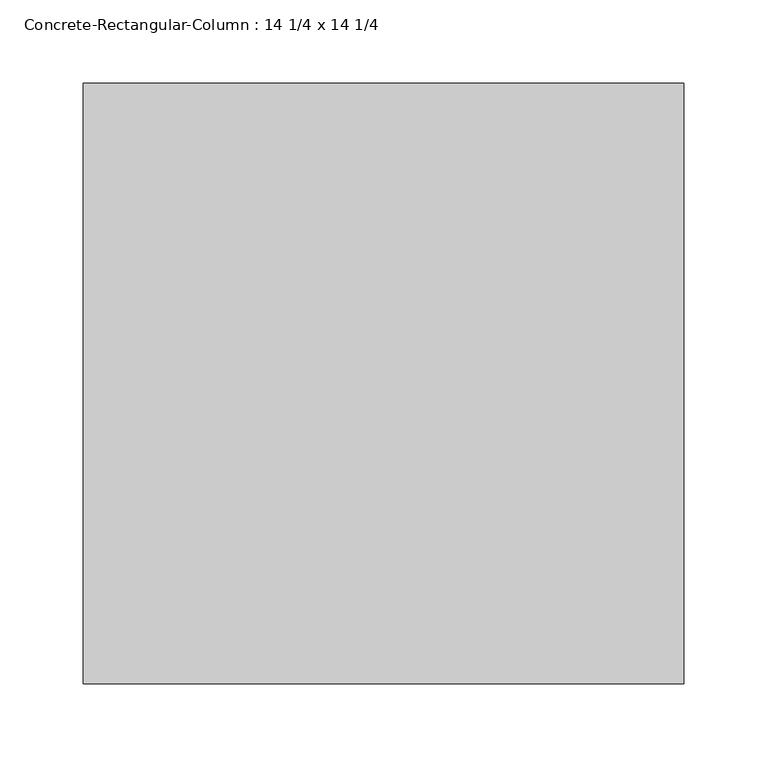
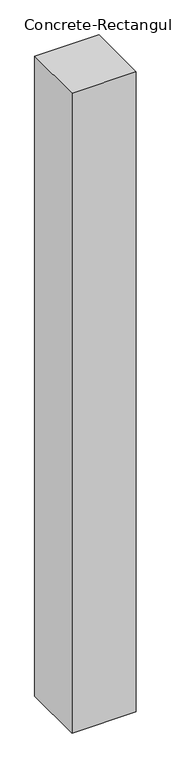
"""IFC4 building model written with IfcOpenShell, lengths in millimetres: column geometry, Concrete-Rectangular-Column : 14 1/4 x 14 1/4."""

import ifcopenshell
import ifcopenshell.guid

model = None  # the IFC model being written
_history = None  # IfcOwnerHistory: only IFC2X3 demands one
_inside = {}  # id of a spatial element -> (the spatial element, [elements in it])
_under = {}  # id of a project, library or spatial element -> (it, [spatial elements below it])
_declared = {}  # id of a project -> (the project, [libraries it declares])
_typed = {}  # id of a type object -> (the type object, [elements of that type])
_made_of = {}  # id of a material, layer set ... -> (it, [elements and type objects made of it])


def new_model(schema):
    """Start an empty IFC model of exactly this schema.

    Asked for "IFC4X3", IfcOpenShell would pick the latest addendum, in which some entities
    have other attributes; the version numbers below select the first issue.
    IFC2X3 requires an IfcOwnerHistory on every rooted entity: one is made here for all.
    """
    global model, _history
    if schema == "IFC4X3":
        model = ifcopenshell.file(schema_version=(4, 3, 0, 0))
    else:
        model = ifcopenshell.file(schema=schema)
    _inside.clear()
    _under.clear()
    _declared.clear()
    _typed.clear()
    _made_of.clear()
    _history = None
    if model.schema == "IFC2X3":
        org = make("IfcOrganization", Name="unknown")
        user = make(
            "IfcPersonAndOrganization",
            ThePerson=make("IfcPerson", FamilyName="unknown"),
            TheOrganization=org,
        )
        app = make(
            "IfcApplication",
            ApplicationDeveloper=org,
            Version="unknown",
            ApplicationFullName="unknown",
            ApplicationIdentifier="unknown",
        )
        _history = make(
            "IfcOwnerHistory",
            OwningUser=user,
            OwningApplication=app,
            ChangeAction="ADDED",
            CreationDate=0,
        )
    return model


def make(cls, **values):
    """One entity of the class cls with the attributes given. An attribute that is None is left unset."""
    return model.create_entity(
        cls, **{name: value for name, value in values.items() if value is not None}
    )


def rooted(cls, **values):
    """An entity with a GlobalId (a new one), such as an element, a storey or a relation."""
    return make(cls, GlobalId=ifcopenshell.guid.new(), OwnerHistory=_history, **values)


def si_unit(unit_type, name, prefix=None):
    """IfcSIUnit, for example si_unit("LENGTHUNIT", "METRE", prefix="MILLI")."""
    return make("IfcSIUnit", UnitType=unit_type, Prefix=prefix, Name=name)


def assignment(units):
    """IfcUnitAssignment: the units of a project."""
    return None if units is None else make("IfcUnitAssignment", Units=units)


def point(xyz):
    """IfcCartesianPoint."""
    return None if xyz is None else make("IfcCartesianPoint", Coordinates=xyz)


def direction(xyz):
    """IfcDirection."""
    return None if xyz is None else make("IfcDirection", DirectionRatios=xyz)


def frame(location, z_axis=None, x_axis=None):
    """IfcAxis2Placement3D, a coordinate frame: its origin and axes. An axis left out is left unset."""
    return make(
        "IfcAxis2Placement3D",
        Location=point(location),
        Axis=direction(z_axis),
        RefDirection=direction(x_axis),
    )


def origin():
    """The frame at (0, 0, 0) with its axes left unset."""
    return frame((0.0, 0.0, 0.0))


def origin_with_axes():
    """The frame at (0, 0, 0) with the z axis (0, 0, 1) and the x axis (1, 0, 0) written out."""
    return frame((0.0, 0.0, 0.0), z_axis=(0.0, 0.0, 1.0), x_axis=(1.0, 0.0, 0.0))


def place(relative_to, where):
    """IfcLocalPlacement: puts the frame where relative to a parent placement (None: the world)."""
    return make(
        "IfcLocalPlacement", PlacementRelTo=relative_to, RelativePlacement=where
    )


def context(
    kind, dimensions, precision=None, world=None, true_north=None, identifier=None
):
    """IfcGeometricRepresentationContext, for example the 3D "Model" context."""
    return make(
        "IfcGeometricRepresentationContext",
        ContextIdentifier=identifier,
        ContextType=kind,
        CoordinateSpaceDimension=dimensions,
        Precision=precision,
        WorldCoordinateSystem=world,
        TrueNorth=true_north,
    )


def project(units=None, contexts=None):
    """IfcProject with its units and contexts."""
    return rooted(
        "IfcProject",
        Name="project",
        RepresentationContexts=contexts,
        UnitsInContext=assignment(units),
    )


def spatial(cls, under=None, at=None, **own):
    """A site, building, storey or space (cls), placed at a placement, below another one or the project."""
    s = rooted(cls, ObjectPlacement=at, **own)
    if under is not None:
        _under.setdefault(under.id(), (under, []))[1].append(s)
    return s


def polyline(points):
    """IfcPolyline through the points."""
    return make("IfcPolyline", Points=[point(p) for p in points])


def outline(outer, holes=None, kind="AREA"):
    """IfcArbitraryClosedProfileDef: a profile drawn as a closed curve; with holes, ...WithVoids."""
    if holes is None:
        return make("IfcArbitraryClosedProfileDef", ProfileType=kind, OuterCurve=outer)
    return make(
        "IfcArbitraryProfileDefWithVoids",
        ProfileType=kind,
        OuterCurve=outer,
        InnerCurves=holes,
    )


def extrude(swept, where, along, depth):
    """IfcExtrudedAreaSolid: the profile swept, set in the frame where, extruded along a direction by depth."""
    return make(
        "IfcExtrudedAreaSolid",
        SweptArea=swept,
        Position=where,
        ExtrudedDirection=direction(along),
        Depth=depth,
    )


def shape(context_of_items, identifier, shape_type, items):
    """IfcShapeRepresentation: the items that make up one representation, for example the "Body"."""
    return make(
        "IfcShapeRepresentation",
        ContextOfItems=context_of_items,
        RepresentationIdentifier=identifier,
        RepresentationType=shape_type,
        Items=items,
    )


def source(mapping_origin, context_of_items, identifier, shape_type, items):
    """IfcRepresentationMap: a shape defined once, which mapped items show again and again."""
    return make(
        "IfcRepresentationMap",
        MappingOrigin=mapping_origin,
        MappedRepresentation=shape(context_of_items, identifier, shape_type, items),
    )


def transform(
    local_origin,
    x_axis=None,
    y_axis=None,
    z_axis=None,
    scale=None,
    scale2=None,
    scale3=None,
    uniform=True,
):
    """IfcCartesianTransformationOperator3D, or its non-uniform kind. x_axis, y_axis, z_axis: its Axis1, 2, 3."""
    if uniform:
        return make(
            "IfcCartesianTransformationOperator3D",
            Axis1=direction(x_axis),
            Axis2=direction(y_axis),
            LocalOrigin=point(local_origin),
            Scale=scale,
            Axis3=direction(z_axis),
        )
    return make(
        "IfcCartesianTransformationOperator3DnonUniform",
        Axis1=direction(x_axis),
        Axis2=direction(y_axis),
        LocalOrigin=point(local_origin),
        Scale=scale,
        Axis3=direction(z_axis),
        Scale2=scale2,
        Scale3=scale3,
    )


def mapped(mapping_source, mapping_target):
    """IfcMappedItem: shows the shape of a source again, moved by a transform."""
    return make(
        "IfcMappedItem", MappingSource=mapping_source, MappingTarget=mapping_target
    )


def made_of(thing, what):
    """Note that an element or type object is made of a material, layer set ...; save() writes the relation."""
    if what is not None:
        _made_of.setdefault(what.id(), (what, []))[1].append(thing)
    return thing


def element(
    cls,
    number,
    at=None,
    inside=None,
    cuts=None,
    type_object=None,
    material=None,
    context=None,
    identifier="Body",
    shape_type=None,
    held_by="IfcProductDefinitionShape",
    body=None,
    shapes=None,
    **own,
):
    """One element of the class cls, such as IfcWall. Its Tag is "e" and its number.

    at: its placement. inside: the storey or other place that contains it. cuts: it is an
    opening in that element (IfcRelVoidsElement). A single representation is given by context,
    identifier, shape_type and body (its items); several are given by shapes. held_by: the class
    of the entity that holds the representations. save() writes the other relations.
    """
    e = rooted(cls, Tag="e%d" % number, ObjectPlacement=at, **own)
    if body is not None:
        shapes = [shape(context, identifier, shape_type, body)]
    if shapes is not None:
        e.Representation = make(held_by, Representations=shapes)
    if inside is not None:
        _inside.setdefault(inside.id(), (inside, []))[1].append(e)
    if cuts is not None:
        rooted(
            "IfcRelVoidsElement", RelatingBuildingElement=cuts, RelatedOpeningElement=e
        )
    if type_object is not None:
        _typed.setdefault(type_object.id(), (type_object, []))[1].append(e)
    return made_of(e, material)


def aggregate(whole, parts):
    """IfcRelAggregates: a whole, such as a stair, and the parts it consists of."""
    return rooted("IfcRelAggregates", RelatingObject=whole, RelatedObjects=parts)


def save(model, path):
    """Write the relations noted so far, then the file.

    IfcRelAggregates (storeys below a building ...), IfcRelContainedInSpatialStructure (elements
    in a storey), IfcRelDefinesByType, IfcRelAssociatesMaterial and IfcRelDeclares: one each for
    every whole, place, type object, material and project.
    """
    for whole, parts in _under.values():
        aggregate(whole, parts)
    for where, things in _inside.values():
        rooted(
            "IfcRelContainedInSpatialStructure",
            RelatedElements=things,
            RelatingStructure=where,
        )
    for kind, things in _typed.values():
        rooted("IfcRelDefinesByType", RelatedObjects=things, RelatingType=kind)
    for what, things in _made_of.values():
        rooted("IfcRelAssociatesMaterial", RelatedObjects=things, RelatingMaterial=what)
    for by, libraries in _declared.values():
        rooted("IfcRelDeclares", RelatingContext=by, RelatedDefinitions=libraries)
    model.write(path)


def concrete_rectangular_column_14_1_4_x_14_1_4_7611fc2a(model_context):
    return source(origin(), model_context, "Body", "SweptSolid", [
        extrude(outline(polyline([(180.975, 180.975), (180.975, -180.975), (-180.975, -180.975), (-180.975, 180.975), (180.975, 180.975)])), origin_with_axes(), (0.0, 0.0, 1.0), 3810.0),
    ])


if __name__ == "__main__":
    model = new_model("IFC4")
    model_context = context("Model", 3, world=origin())
    ifc_project = project(units=[si_unit("LENGTHUNIT", "METRE", prefix="MILLI")], contexts=[model_context])
    site = spatial("IfcSite", under=ifc_project)
    building = spatial("IfcBuilding", under=site)
    placement = place(None, origin())
    concrete_rectangular_column_14_1_4_x_14_1_4_shape = concrete_rectangular_column_14_1_4_x_14_1_4_7611fc2a(model_context)
    element("IfcColumn", 1, ObjectType="Concrete-Rectangular-Column : 14 1/4 x 14 1/4", at=placement, inside=building, context=model_context, shape_type="MappedRepresentation", body=[
        mapped(concrete_rectangular_column_14_1_4_x_14_1_4_shape, transform((0.0, 0.0, 0.0), x_axis=(1.0, 0.0, 0.0), y_axis=(0.0, 1.0, 0.0), z_axis=(0.0, 0.0, 1.0))),
    ])
    save(model, "model.ifc")

# Revit data of these elements
# Type "Concrete-Rectangular-Column : 14 1/4 x 14 1/4"
#   Assembly Code = "B10"
#   b = 361.95 mm
#   h = 361.95 mm
#   Structural Material [instance default] = Concrete - Cast-in-Place Concrete
# Element 1 (IfcColumn, "Concrete-Rectangular-Column : 14 1/4 x 14 1/4")
#   Materials on its faces: "Concrete - Cast-in-Place Concrete"
# Materials
#   "Concrete - Cast-in-Place Concrete": class "Concrete", colour RGB 192 192 192, transparency 0
